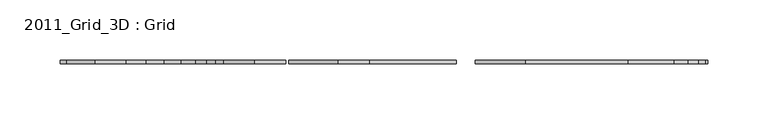
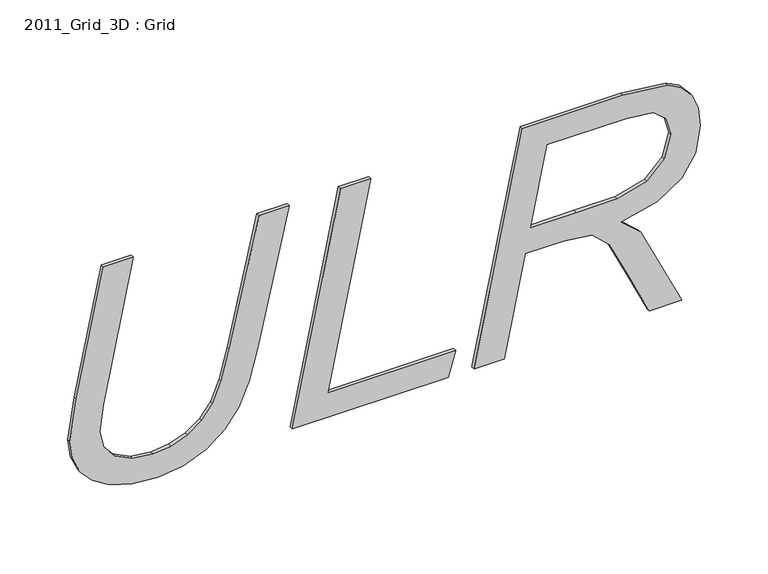
"""IFC4 building model written with IfcOpenShell, lengths in millimetres: proxy geometry, 2011_Grid_3D : Grid."""

from ifc_helpers import new_model, si_unit, frame, origin, place, context, project, spatial, polyline, outline, extrude, source, transform, mapped, element, save


def proxy_2011_grid_3d_grid_369c63fd(model_context):
    return source(origin(), model_context, "Body", "SweptSolid", [
        extrude(outline(polyline([(101.4447294, 47277.8299768), (-9.5457855, 47254.7296731), (-46.3278141, 47249.0785258), (-62.2836301, 47251.2224918), (-76.4424804, 47257.6543897), (-88.2714718, 47268.3866123), (-97.2377109, 47283.4315526), (-102.8888581, 47302.2191386), (-104.7725739, 47324.1792986), (-102.1081075, 47346.374923), (-94.1147085, 47365.6706165), (-81.7032524, 47381.5706646), (-65.784615, 47393.5793525), (-44.9584024, 47402.6757168), (-17.8242205, 47409.8387938), (101.4447294, 47437.0039577), (101.4447294, 47411.0780804), (-10.7355007, 47385.4992034), (-36.7791103, 47378.8070553), (-54.6310349, 47371.3217638), (-66.7202764, 47362.0271137), (-75.4758368, 47349.90689), (-80.7923767, 47335.8285933), (-82.5645566, 47320.6597244), (-80.0983761, 47302.5599424), (-72.6998347, 47287.8186274), (-61.2488258, 47278.0220662), (-46.6252429, 47274.7565458), (-23.5745107, 47277.8795482), (101.4447294, 47303.5575682), (101.4447294, 47277.8299768)])), frame((0.0, -3.175, 0.0), z_axis=(0.0, 1.0, 0.0), x_axis=(0.0, 0.0, 1.0)), (0.0, 0.0, 1.0), 3.175),
        extrude(outline(polyline([(-101.6, 47439.4329596), (-101.6, 47572.6810633), (-79.3919827, 47579.0262111), (-79.3919827, 47469.7211261), (101.4447294, 47506.4535832), (101.4447294, 47480.6764203), (-101.6, 47439.4329596)])), frame((0.0, -3.175, 0.0), z_axis=(0.0, 1.0, 0.0), x_axis=(0.0, 0.0, 1.0)), (0.0, 0.0, 1.0), 3.175),
        extrude(outline(polyline([(-101.6, 47594.8890806), (-101.6, 47620.6662435), (-12.7679309, 47638.7102575), (-12.7679309, 47671.5761402), (-15.9652905, 47695.9405163), (-29.4239439, 47710.3410275), (-64.4213996, 47727.0466119), (-101.6, 47744.7931972), (-101.6, 47772.5036473), (-64.6196855, 47754.856205), (-27.4906566, 47737.1591912), (-12.7679309, 47720.4536068), (-4.8736748, 47751.3490237), (8.8948002, 47772.3549329), (27.7567435, 47784.4007994), (50.9314044, 47788.4160883), (67.4758815, 47786.5509618), (80.922142, 47780.9555825), (90.9231855, 47772.0822898), (97.1320117, 47760.3834236), (101.4447294, 47721.8911794), (101.4447294, 47636.1325412), (-101.6, 47594.8890806)]), holes=[polyline([(9.4400864, 47643.221261), (79.2367121, 47657.3987006), (79.2367121, 47725.3611821), (76.8077102, 47748.1144855), (67.6122031, 47758.9210653), (51.7245478, 47763.0354971), (31.524175, 47757.6322072), (16.5783776, 47742.4385525), (9.4400864, 47717.2810329), (9.4400864, 47682.1348627), (9.4400864, 47643.221261)])]), frame((0.0, -3.175, 0.0), z_axis=(0.0, 1.0, 0.0), x_axis=(0.0, 0.0, 1.0)), (0.0, 0.0, 1.0), 3.175),
    ])


if __name__ == "__main__":
    model = new_model("IFC4")
    model_context = context("Model", 3, world=origin())
    ifc_project = project(units=[si_unit("LENGTHUNIT", "METRE", prefix="MILLI")], contexts=[model_context])
    site = spatial("IfcSite", under=ifc_project)
    building = spatial("IfcBuilding", under=site)
    placement = place(None, origin())
    proxy_2011_grid_3d_grid_shape = proxy_2011_grid_3d_grid_369c63fd(model_context)
    element("IfcBuildingElementProxy", 1, Name="2011_Grid_3D : Grid", ObjectType="2011_Grid_3D : Grid", at=placement, inside=building, context=model_context, shape_type="MappedRepresentation", body=[
        mapped(proxy_2011_grid_3d_grid_shape, transform((0.0, 0.0, 0.0), x_axis=(1.0, 0.0, 0.0), y_axis=(0.0, 1.0, 0.0), z_axis=(0.0, 0.0, 1.0))),
    ])
    save(model, "model.ifc")

# Revit data of these elements
# Type "2011_Grid_3D : Grid"
#   Workplane [instance default] = "LEVEL"
#   Grid [instance default] = "S"
#   t [instance default] = 12' - 6"
#   built-in parameter 1001306 [instance default] = 50 (stored number, unit not read)
#   d [instance default] = 2
#   Symbol At End 2 [instance default] = yes
#   Symbol At End 1 [instance default] = yes
#   Robust [instance default] = yes
#   No of grid markers [instance default] = 3
#   Grid Height Visible = yes
#   Height = 0
#   Assembly Code = ""
# Element 1 (IfcBuildingElementProxy, "2011_Grid_3D : Grid")
#   Workplane = "ULR"
#   Grid = "A"
#   t = 11' - 0.37148"
#   built-in parameter 1001306 = 154.433 (stored number, unit not read)
#   d = 7
#   Robust = no
#   No of grid markers = 8
#   Materials on its faces: "Letter"
# Materials
#   "Letter": class "Unassigned", colour RGB 178 187 30, transparency 0, Comments = "Rendering appearance not upgraded "
